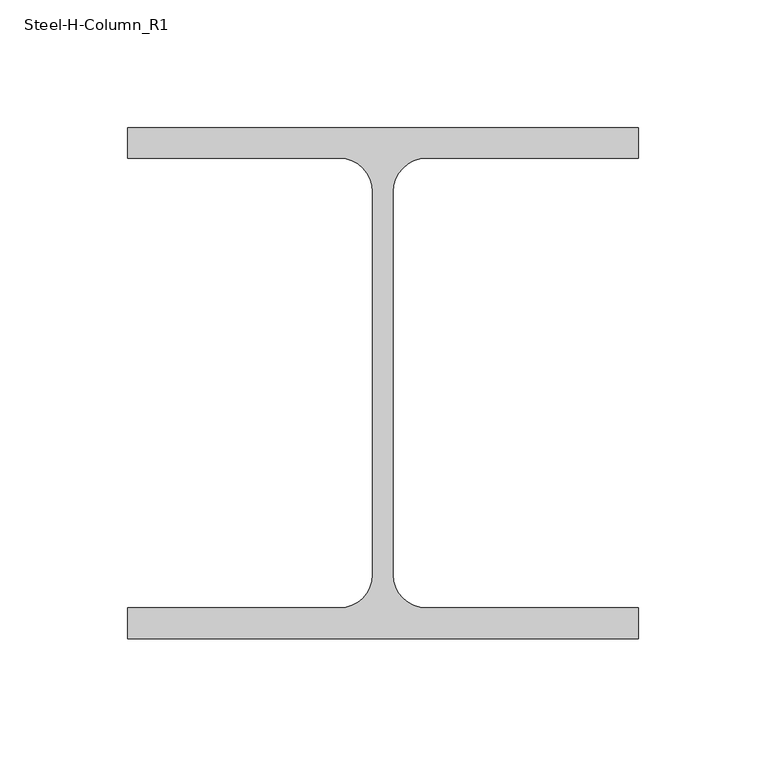
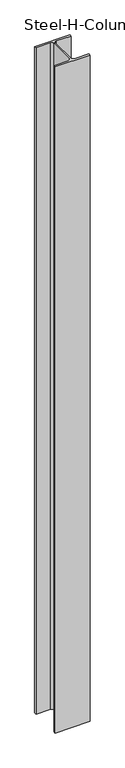
"""IFC4 building model written with IfcOpenShell, lengths in millimetres: column geometry, Steel-H-Column_R1 : CL121_H-200×200x8x12."""

from ifc_helpers import new_model, si_unit, point, frame, frame_2d, origin, place, context, project, spatial, polyline, circle_curve, trimmed, segment, composite_curve, outline, extrude, source, transform, mapped, element, save


def steel_h_column_r1_5833ab44(model_context):
    return source(origin(), model_context, "Body", "SweptSolid", [
        extrude(outline(composite_curve([segment(polyline([(100.0, 100.0), (100.0, 88.0), (17.0, 88.0)]), True, "CONTINUOUS"), segment(trimmed(circle_curve(frame_2d((17.0, 75.0)), 13.0), [point((17.0, 88.0))], [point((4.0, 75.0))], True, "CARTESIAN"), True, "CONTINUOUS"), segment(polyline([(4.0, 75.0), (4.0, -75.0)]), True, "CONTINUOUS"), segment(trimmed(circle_curve(frame_2d((17.0, -75.0)), 13.0), [point((4.0, -75.0))], [point((17.0, -88.0))], True, "CARTESIAN"), True, "CONTINUOUS"), segment(polyline([(17.0, -88.0), (100.0, -88.0), (100.0, -100.0), (-100.0, -100.0), (-100.0, -88.0), (-17.0, -88.0)]), True, "CONTINUOUS"), segment(trimmed(circle_curve(frame_2d((-17.0, -75.0)), 13.0), [point((-17.0, -88.0))], [point((-4.0, -75.0))], True, "CARTESIAN"), True, "CONTINUOUS"), segment(polyline([(-4.0, -75.0), (-4.0, 75.0)]), True, "CONTINUOUS"), segment(trimmed(circle_curve(frame_2d((-17.0, 75.0)), 13.0), [point((-4.0, 75.0))], [point((-17.0, 88.0))], True, "CARTESIAN"), True, "CONTINUOUS"), segment(polyline([(-17.0, 88.0), (-100.0, 88.0), (-100.0, 100.0), (100.0, 100.0)]), True, "CONTINUOUS")], self_intersect=False)), frame((0.0, 0.0, 50.0), z_axis=(0.0, 0.0, 1.0), x_axis=(1.0, 0.0, 0.0)), (0.0, 0.0, 1.0), 4000.0),
    ])


if __name__ == "__main__":
    model = new_model("IFC4")
    model_context = context("Model", 3, world=origin())
    ifc_project = project(units=[si_unit("LENGTHUNIT", "METRE", prefix="MILLI")], contexts=[model_context])
    site = spatial("IfcSite", under=ifc_project)
    building = spatial("IfcBuilding", under=site)
    placement = place(None, origin())
    steel_h_column_r1_shape = steel_h_column_r1_5833ab44(model_context)
    element("IfcColumn", 1, ObjectType="Steel-H-Column_R1 : CL121_H-200×200x8x12", at=placement, inside=building, context=model_context, shape_type="MappedRepresentation", body=[
        mapped(steel_h_column_r1_shape, transform((0.0, 0.0, 0.0), x_axis=(1.0, 0.0, 0.0), y_axis=(0.0, 1.0, 0.0), z_axis=(0.0, 0.0, 1.0))),
    ])
    save(model, "model.ifc")

# Revit data of these elements
# Type "Steel-H-Column_R1 : CL121_H-200×200x8x12"
#   Surface Area = 1.16168 m²/m
#   Section Area = 63.5307 cm²
#   Mass per Unit Length = 49.8716 kg/m
#   B = 200 mm
#   H = 200 mm
#   r = 13 mm
#   tw = 8 mm
#   tf = 12 mm
#   hec_material4 [instance default] = none
#   hec_material2 [instance default] = none
#   hec_material1 [instance default] = none
#   hec_material3 [instance default] = none
#   Structural Material [instance default] = Steel, 45-345
#   Assembly Code = ""
# Element 1 (IfcColumn, "Steel-H-Column_R1 : CL121_H-200×200x8x12")
#   Structural Material = none
# Materials
#   "Steel, 45-345": class "Metal", colour RGB 189 187 185, transparency 0, Description = "Steel 345 MPa", Cost = 0
